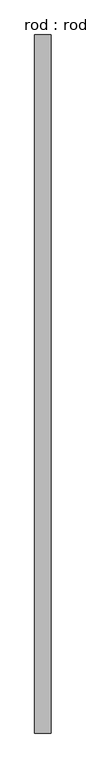
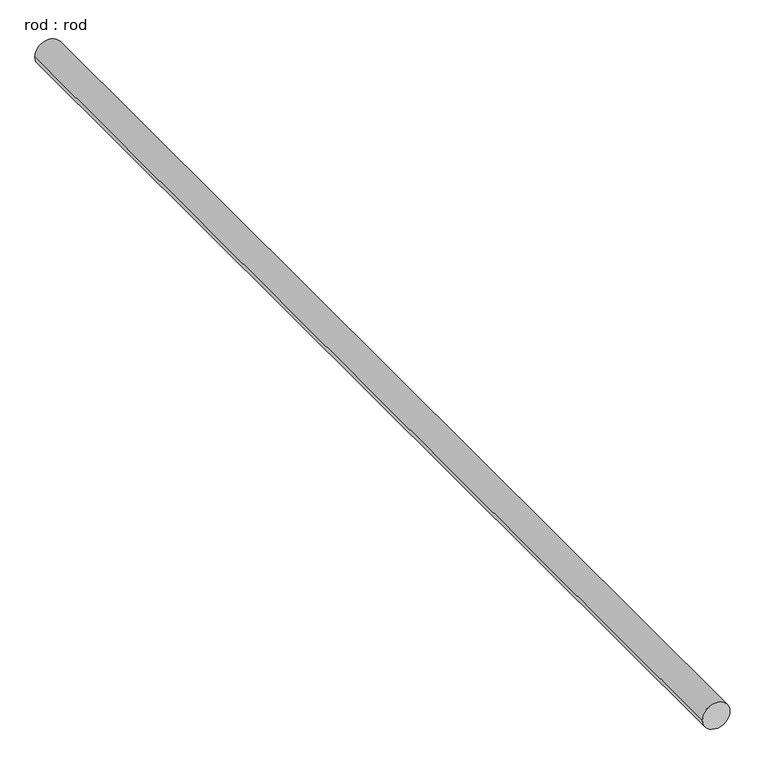
"""IFC4 building model written with IfcOpenShell, lengths in millimetres: proxy geometry, rod : rod."""

from ifc_helpers import new_model, si_unit, point, frame, frame_2d, origin, place, context, project, spatial, circle_curve, trimmed, segment, composite_curve, outline, extrude, source, transform, mapped, element, save


def rod_rod_0ade6199(model_context):
    return source(origin(), model_context, "Body", "SweptSolid", [
        extrude(outline(composite_curve([segment(trimmed(circle_curve(frame_2d((0.0108462, 0.0)), 200.0), [point((0.0108462, 200.0))], [point((0.0108462, -200.0))], False, "CARTESIAN"), True, "CONTINUOUS"), segment(trimmed(circle_curve(frame_2d((0.0108462, 0.0)), 200.0), [point((0.0108462, -200.0))], [point((0.0108462, 200.0))], False, "CARTESIAN"), True, "CONTINUOUS")], self_intersect=False)), frame((0.0, -4344.7713847, 0.0), z_axis=(0.0, 1.0, 0.0), x_axis=(0.0, 0.0, 1.0)), (0.0, 0.0, 1.0), 16875.0),
    ])


if __name__ == "__main__":
    model = new_model("IFC4")
    model_context = context("Model", 3, world=origin())
    ifc_project = project(units=[si_unit("LENGTHUNIT", "METRE", prefix="MILLI")], contexts=[model_context])
    site = spatial("IfcSite", under=ifc_project)
    building = spatial("IfcBuilding", under=site)
    placement = place(None, origin())
    rod_rod_shape = rod_rod_0ade6199(model_context)
    element("IfcBuildingElementProxy", 1, Name="rod : rod", ObjectType="rod : rod", at=placement, inside=building, context=model_context, shape_type="MappedRepresentation", body=[
        mapped(rod_rod_shape, transform((0.0, 0.0, 0.0), x_axis=(1.0, 0.0, 0.0), y_axis=(0.0, 1.0, 0.0), z_axis=(0.0, 0.0, 1.0))),
    ])
    save(model, "model.ifc")

# Revit data of these elements
# Type "rod : rod"
#   Default Elevation = 0
